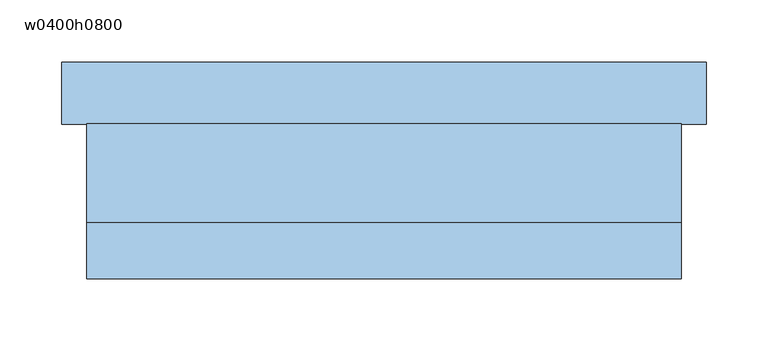
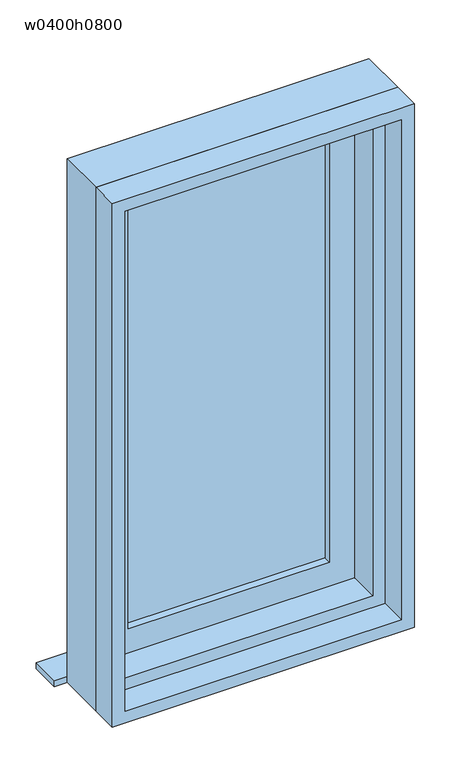
"""IFC4 building model written with IfcOpenShell, lengths in millimetres: window geometry, 縦すべり窓 : w0400h0800."""

from ifc_helpers import new_model, si_unit, frame, origin, place, context, project, spatial, polyline, outline, extrude, source, transform, mapped, element, save


def w0400h0800_0b9f01bb(model_context):
    return source(origin(), model_context, "Body", "SweptSolid", [
        extrude(outline(polyline([(160.0, 22.5), (-160.0, 22.5), (-160.0, 27.5), (160.0, 27.5), (160.0, 22.5)])), frame((0.0, 0.0, 1240.0), z_axis=(0.0, 0.0, 1.0), x_axis=(1.0, 0.0, 0.0)), (0.0, 0.0, 1.0), 720.0),
        extrude(outline(polyline([(2000.0, 200.0), (2000.0, -200.0), (1200.0, -200.0), (1200.0, 200.0), (2000.0, 200.0)]), holes=[polyline([(1960.0, -160.0), (1960.0, 160.0), (1240.0, 160.0), (1240.0, -160.0), (1960.0, -160.0)])]), frame((0.0, 10.0, 0.0), z_axis=(0.0, 1.0, 0.0), x_axis=(0.0, 0.0, 1.0)), (0.0, 0.0, 1.0), 30.0),
        extrude(outline(polyline([(260.0, 90.0), (260.0, 40.0), (-260.0, 40.0), (-260.0, 90.0), (260.0, 90.0)])), frame((0.0, 0.0, 1160.0), z_axis=(0.0, 0.0, 1.0), x_axis=(1.0, 0.0, 0.0)), (0.0, 0.0, 1.0), 10.0),
        extrude(outline(polyline([(2040.0, 240.0), (2040.0, -240.0), (1160.0, -240.0), (1160.0, 240.0), (2040.0, 240.0)]), holes=[polyline([(1180.0, -220.0), (2020.0, -220.0), (2020.0, 220.0), (1180.0, 220.0), (1180.0, -220.0)])]), frame((0.0, -85.0, 0.0), z_axis=(0.0, 1.0, 0.0), x_axis=(0.0, 0.0, 1.0)), (0.0, 0.0, 1.0), 45.0),
        extrude(outline(polyline([(2040.0, -240.0), (1160.0, -240.0), (1160.0, 240.0), (2040.0, 240.0), (2040.0, -240.0)]), holes=[polyline([(2000.0, 200.0), (1200.0, 200.0), (1200.0, -200.0), (2000.0, -200.0), (2000.0, 200.0)])]), frame((0.0, -40.0, 0.0), z_axis=(0.0, 1.0, 0.0), x_axis=(0.0, 0.0, 1.0)), (0.0, 0.0, 1.0), 80.0),
    ])


if __name__ == "__main__":
    model = new_model("IFC4")
    model_context = context("Model", 3, world=origin())
    ifc_project = project(units=[si_unit("LENGTHUNIT", "METRE", prefix="MILLI")], contexts=[model_context])
    site = spatial("IfcSite", under=ifc_project)
    building = spatial("IfcBuilding", under=site)
    placement = place(None, origin())
    w0400h0800_shape = w0400h0800_0b9f01bb(model_context)
    element("IfcWindow", 1, ObjectType="縦すべり窓 : w0400h0800", at=placement, inside=building, context=model_context, shape_type="MappedRepresentation", body=[
        mapped(w0400h0800_shape, transform((0.0, 0.0, 0.0), x_axis=(1.0, 0.0, 0.0), y_axis=(0.0, 1.0, 0.0), z_axis=(0.0, 0.0, 1.0))),
    ])
    save(model, "model.ifc")

# Revit data of these elements
# Project information
#   プロジェクト発行日 = "発行日"
#   プロジェクト ステータス = "プロジェクト ステータス"
#   クライアント名 = "オーナ"
#   計画地住所 = "ここにアドレスを入力"
#   プロジェクト名 = "プロジェクト名"
#   プロジェクト番号 = "0001"
# Type "縦すべり窓 : w0400h0800"
#   Construction Type Id = "GSP4R"
#   Analytic Construction = "1/8 インチ ピルキントン一重ガラス"
#   Type Mark = "84"
#   Operation = "シングルパネル"
#   Keynote = "08520.S3"
#   Visual Light Transmittance = 0.9
#   Solar Heat Gain Coefficient = 0.86
#   Heat Transfer Coefficient (U) = 6.7069 W/(m²·K)
#   Height = 800 mm
#   既定の腰高 = 1200 mm
#   Width = 400 mm
#   額縁見附 = 20 mm
#   額縁ちり = 10 mm
#   サッシ見附 = 40 mm
#   サッシの幅 = 80 mm
#   サッシ額縁 [instance default] = none
#   サッシ本体 [instance default] = none
#   サッシガラス [instance default] = ガラス - 透明
#   Wall Closure = (empty or 0)
#   Type Comments = ""
#   Assembly Code = ""
# Element 1 (IfcWindow, "縦すべり窓 : w0400h0800")
#   Materials on its faces: "ガラス - 透明"
# Materials
#   "ガラス - 透明": class "ガラス", colour RGB 0 128 192, transparency 0.9, Cost = 0
